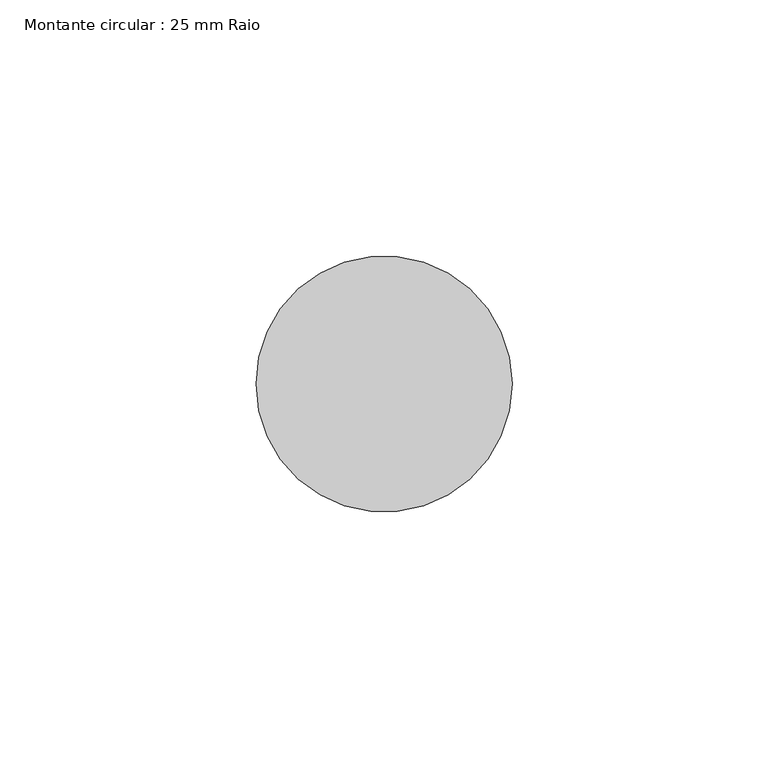
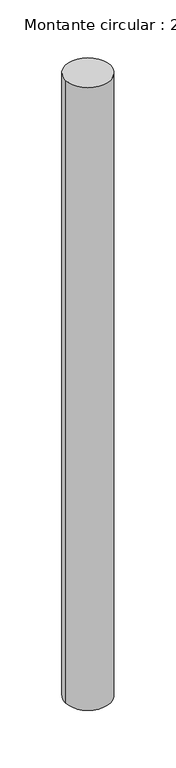
"""IFC4 building model written with IfcOpenShell, lengths in millimetres: member geometry, Montante circular : 25 mm Raio."""

from ifc_helpers import new_model, si_unit, point, frame, frame_2d, origin, place, context, project, spatial, circle_curve, trimmed, segment, composite_curve, outline, extrude, source, transform, mapped, element, save


def montante_circular_25_mm_raio_f24612f6(model_context):
    return source(origin(), model_context, "Body", "SweptSolid", [
        extrude(outline(composite_curve([segment(trimmed(circle_curve(frame_2d((-25.0, 0.0)), 25.0), [point((0.0, 0.0))], [point((-50.0, 0.0))], False, "CARTESIAN"), True, "CONTINUOUS"), segment(trimmed(circle_curve(frame_2d((-25.0, 0.0)), 25.0), [point((-50.0, 0.0))], [point((0.0, 0.0))], False, "CARTESIAN"), True, "CONTINUOUS")], self_intersect=False)), frame((0.0, 0.0, -727.4383788), z_axis=(0.0, 0.0, 1.0), x_axis=(1.0, 0.0, 0.0)), (0.0, 0.0, 1.0), 727.4383788),
    ])


if __name__ == "__main__":
    model = new_model("IFC4")
    model_context = context("Model", 3, world=origin())
    ifc_project = project(units=[si_unit("LENGTHUNIT", "METRE", prefix="MILLI")], contexts=[model_context])
    site = spatial("IfcSite", under=ifc_project)
    building = spatial("IfcBuilding", under=site)
    placement = place(None, origin())
    montante_circular_25_mm_raio_shape = montante_circular_25_mm_raio_f24612f6(model_context)
    element("IfcMember", 1, ObjectType="Montante circular : 25 mm Raio", at=placement, inside=building, context=model_context, shape_type="MappedRepresentation", body=[
        mapped(montante_circular_25_mm_raio_shape, transform((0.0, 0.0, 0.0), x_axis=(1.0, 0.0, 0.0), y_axis=(0.0, 1.0, 0.0), z_axis=(0.0, 0.0, 1.0))),
    ])
    save(model, "model.ifc")

# Revit data of these elements
# Type "Montante circular : 25 mm Raio"
#   built-in parameter 1007350 = 0.082021 (stored number, unit not read)
# Element 1 (IfcMember, "Montante circular : 25 mm Raio")
#   Materials on its faces: "Alumín."
# Materials
#   "Alumín.": class "Metal", colour RGB 247 247 247, transparency 0, Description = "Alumín. 6061", Cost = 0
